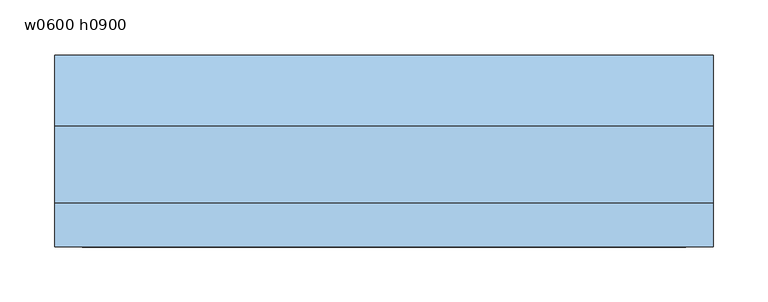
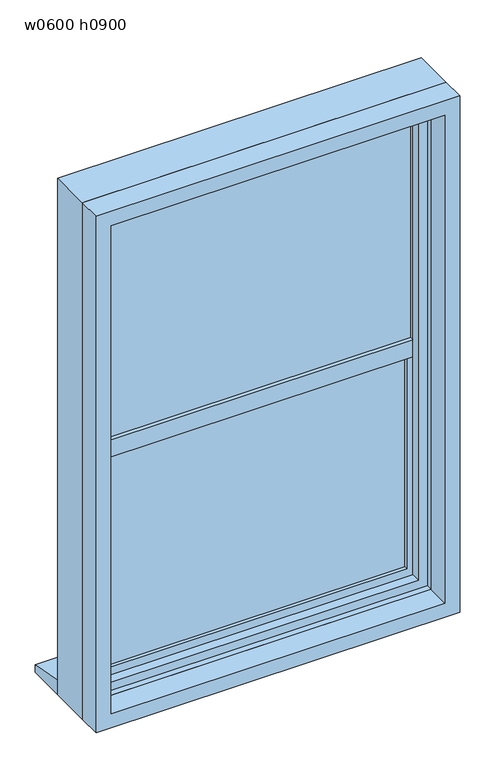
"""IFC4 building model written with IfcOpenShell, lengths in millimetres: window geometry, 上げ下げ窓 : w0600 h0900."""

from ifc_helpers import new_model, si_unit, frame, origin, place, context, project, spatial, polyline, outline, extrude, faceted_brep, source, transform, mapped, element, save


def w0600_h0900_44770d6e(model_context):
    return source(origin(), model_context, "Body", "SolidModel", [
        faceted_brep([(-300.0, -45.0, 1700.0), (-300.0, 25.0, 1700.0), (-300.0, 25.0, 800.0), (-300.0, -45.0, 800.0), (300.0, 25.0, 1700.0), (300.0, 25.0, 800.0), (-275.0, 25.0, 825.0), (275.0, 25.0, 825.0), (275.0, 25.0, 1675.0), (-275.0, 25.0, 1675.0), (300.0, -45.0, 800.0), (300.0, -45.0, 1700.0), (-275.0, -45.0, 1675.0), (275.0, -45.0, 1675.0), (275.0, -45.0, 825.0), (-275.0, -45.0, 825.0), (-275.0, -35.0, 1675.0), (-275.0, -35.0, 825.0), (275.0, -35.0, 825.0), (275.0, -35.0, 1675.0), (-260.0, -35.0, 1660.0), (260.0, -35.0, 1660.0), (260.0, -35.0, 840.0), (-260.0, -35.0, 840.0), (-260.0, -20.0, 1660.0), (-260.0, -20.0, 840.0), (260.0, -20.0, 840.0), (-275.0, -20.0, 1675.0), (275.0, -20.0, 1675.0), (275.0, -20.0, 825.0), (-275.0, -20.0, 825.0), (260.0, -20.0, 1660.0)], [[[0, 1, 2, 3]], [[1, 4, 5, 2], [6, 7, 8, 9]], [[3, 2, 5, 10]], [[3, 10, 11, 0], [12, 13, 14, 15]], [[16, 12, 15, 17]], [[17, 15, 14, 18]], [[17, 18, 19, 16], [20, 21, 22, 23]], [[24, 20, 23, 25]], [[25, 23, 22, 26]], [[27, 28, 29, 30], [25, 26, 31, 24]], [[9, 27, 30, 6]], [[6, 30, 29, 7]], [[10, 5, 4, 11]], [[18, 14, 13, 19]], [[26, 22, 21, 31]], [[7, 29, 28, 8]], [[11, 4, 1, 0]], [[19, 13, 12, 16]], [[31, 21, 20, 24]], [[8, 28, 27, 9]]]),
        extrude(outline(polyline([(1700.0, 300.0), (1700.0, -300.0), (800.0, -300.0), (800.0, 300.0), (1700.0, 300.0)]), holes=[polyline([(825.0, 275.0), (825.0, -275.0), (1675.0, -275.0), (1675.0, 275.0), (825.0, 275.0)])]), frame((0.0, -85.0, 0.0), z_axis=(0.0, 1.0, 0.0), x_axis=(0.0, 0.0, 1.0)), (0.0, 0.0, 1.0), 40.0),
        extrude(outline(polyline([(260.0, -13.6833097), (-260.0, -13.6833097), (-260.0, -8.6833097), (260.0, -8.6833097), (260.0, -13.6833097)])), frame((0.0, 0.0, 1250.0), z_axis=(0.0, 0.0, 1.0), x_axis=(1.0, 0.0, 0.0)), (0.0, 0.0, 1.0), 410.0),
        extrude(outline(polyline([(-260.0, 8.6833097), (260.0, 8.6833097), (260.0, 3.6833097), (-260.0, 3.6833097), (-260.0, 8.6833097)])), frame((0.0, 0.0, 840.0), z_axis=(0.0, 0.0, 1.0), x_axis=(1.0, 0.0, 0.0)), (0.0, 0.0, 1.0), 380.0),
        extrude(outline(polyline([(1250.0, -275.0), (825.0, -275.0), (825.0, 275.0), (1250.0, 275.0), (1250.0, -275.0)]), holes=[polyline([(840.0, -260.0), (1220.0, -260.0), (1220.0, 260.0), (840.0, 260.0), (840.0, -260.0)])]), frame((0.0, -2.5, 0.0), z_axis=(0.0, 1.0, 0.0), x_axis=(0.0, 0.0, 1.0)), (0.0, 0.0, 1.0), 17.5),
        extrude(outline(polyline([(1220.0, -275.0), (1220.0, 275.0), (1675.0, 275.0), (1675.0, -275.0), (1220.0, -275.0)]), holes=[polyline([(1660.0, -260.0), (1660.0, 260.0), (1250.0, 260.0), (1250.0, -260.0), (1660.0, -260.0)])]), frame((0.0, -20.0, 0.0), z_axis=(0.0, 1.0, 0.0), x_axis=(0.0, 0.0, 1.0)), (0.0, 0.0, 1.0), 17.5),
        extrude(outline(polyline([(90.0, 800.0), (25.0, 800.0), (25.0, 825.0), (90.0, 813.0), (90.0, 800.0)])), frame((-300.0, 0.0, 0.0), z_axis=(1.0, 0.0, 0.0), x_axis=(0.0, 1.0, 0.0)), (0.0, 0.0, 1.0), 600.0),
    ])


if __name__ == "__main__":
    model = new_model("IFC4")
    model_context = context("Model", 3, world=origin())
    ifc_project = project(units=[si_unit("LENGTHUNIT", "METRE", prefix="MILLI")], contexts=[model_context])
    site = spatial("IfcSite", under=ifc_project)
    building = spatial("IfcBuilding", under=site)
    placement = place(None, origin())
    w0600_h0900_shape = w0600_h0900_44770d6e(model_context)
    element("IfcWindow", 1, ObjectType="上げ下げ窓 : w0600 h0900", at=placement, inside=building, context=model_context, shape_type="MappedRepresentation", body=[
        mapped(w0600_h0900_shape, transform((0.0, 0.0, 0.0), x_axis=(1.0, 0.0, 0.0), y_axis=(0.0, 1.0, 0.0), z_axis=(0.0, 0.0, 1.0))),
    ])
    save(model, "model.ifc")

# Revit data of these elements
# Project information
#   プロジェクト発行日 = "発行日"
#   プロジェクト ステータス = "プロジェクト ステータス"
#   クライアント名 = "オーナ"
#   計画地住所 = "ここにアドレスを入力"
#   プロジェクト名 = "プロジェクト名"
#   プロジェクト番号 = "0001"
# Type "上げ下げ窓 : w0600 h0900"
#   Construction Type Id = "GSP4R"
#   Analytic Construction = "1/8 インチ ピルキントン一重ガラス"
#   Type Mark = "100"
#   Operation = "ダブル パネル横"
#   Keynote = "08520.Z1"
#   Visual Light Transmittance = 0.9
#   Solar Heat Gain Coefficient = 0.86
#   Heat Transfer Coefficient (U) = 6.7069 W/(m²·K)
#   Height = 900 mm
#   額縁見附 = 25 mm
#   額縁ちり = 10 mm
#   既定の腰高 = 800 mm
#   Width = 600 mm
#   サッシ枠見附 = 40 mm
#   サッシ枠見込 = 70 mm
#   内枠 = 木目 - ナチュラル
#   サッシ = none
#   ガラス = ガラス - 透明
#   Wall Closure = (empty or 0)
# Element 1 (IfcWindow, "上げ下げ窓 : w0600 h0900")
#   Materials on its faces: "ガラス - 透明", "木目 - ナチュラル"
# Materials
#   "木目 - ナチュラル": class "木材", colour RGB 204 173 122, transparency 0, Cost = 0
#   "ガラス - 透明": class "ガラス", colour RGB 0 128 192, transparency 0.9, Cost = 0
